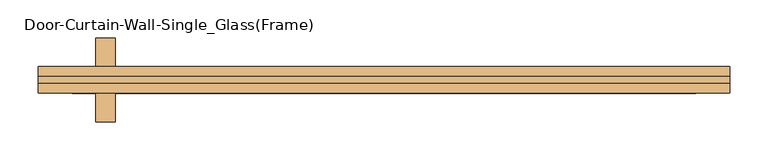
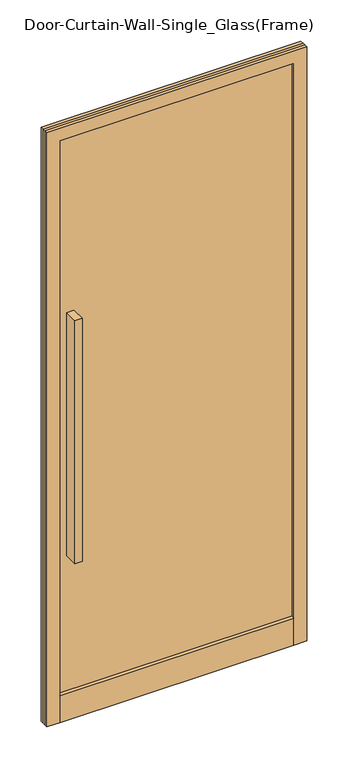
"""IFC4 building model written with IfcOpenShell, lengths in millimetres: door geometry, Door-Curtain-Wall-Single_Glass(Frame) : H_DR_AR B12_Door_Single_Glass_W1000xH2200_SSD-1."""

from ifc_helpers import new_model, si_unit, frame, origin, origin_with_axes, place, context, project, spatial, polyline, outline, extrude, source, transform, mapped, element, save


def door_curtain_wall_single_glass_frame_1226d56c(model_context):
    return source(origin(), model_context, "Body", "SweptSolid", [
        extrude(outline(polyline([(455.0, 0.0), (-455.0, 0.0), (-455.0, 9.0), (455.0, 9.0), (455.0, 0.0)])), origin_with_axes(), (0.0, 0.0, 1.0), 2200.0),
        extrude(outline(polyline([(-353.4, -50.8), (-378.8, -50.8), (-378.8, 0.0), (-353.4, 0.0), (-353.4, -50.8)])), frame((0.0, 0.0, 600.0), z_axis=(0.0, 0.0, 1.0), x_axis=(1.0, 0.0, 0.0)), (0.0, 0.0, 1.0), 900.0),
        extrude(outline(polyline([(-378.8, 59.8), (-353.4, 59.8), (-353.4, 9.0), (-378.8, 9.0), (-378.8, 59.8)])), frame((0.0, 0.0, 600.0), z_axis=(0.0, 0.0, 1.0), x_axis=(1.0, 0.0, 0.0)), (0.0, 0.0, 1.0), 900.0),
        extrude(outline(polyline([(0.0, 410.0), (0.0, 455.0), (2200.0, 455.0), (2200.0, -455.0), (0.0, -455.0), (0.0, -410.0), (2155.0, -410.0), (2155.0, 410.0), (0.0, 410.0)])), frame((0.0, -13.0, 0.0), z_axis=(0.0, 1.0, 0.0), x_axis=(0.0, 0.0, 1.0)), (0.0, 0.0, 1.0), 35.0),
        extrude(outline(polyline([(410.0, 22.0), (410.0, -13.0), (-410.0, -13.0), (-410.0, 22.0), (410.0, 22.0)])), origin_with_axes(), (0.0, 0.0, 1.0), 100.0),
    ])


if __name__ == "__main__":
    model = new_model("IFC4")
    model_context = context("Model", 3, world=origin())
    ifc_project = project(units=[si_unit("LENGTHUNIT", "METRE", prefix="MILLI")], contexts=[model_context])
    site = spatial("IfcSite", under=ifc_project)
    building = spatial("IfcBuilding", under=site)
    placement = place(None, origin())
    door_curtain_wall_single_glass_frame_shape = door_curtain_wall_single_glass_frame_1226d56c(model_context)
    element("IfcDoor", 1, ObjectType="Door-Curtain-Wall-Single_Glass(Frame) : H_DR_AR B12_Door_Single_Glass_W1000xH2200_SSD-1", at=placement, inside=building, context=model_context, shape_type="MappedRepresentation", body=[
        mapped(door_curtain_wall_single_glass_frame_shape, transform((0.0, 0.0, 0.0), x_axis=(1.0, 0.0, 0.0), y_axis=(0.0, 1.0, 0.0), z_axis=(0.0, 0.0, 1.0))),
    ])
    save(model, "model.ifc")

# Revit data of these elements
# Type "Door-Curtain-Wall-Single_Glass(Frame) : H_DR_AR B12_Door_Single_Glass_W1000xH2200_SSD-1"
#   Type Mark = "448"
#   Assembly Code = "B2030100"
#   Analytic Construction = "<None>"
#   Width [instance default] = 914.4 mm
#   Thermal Resistance (R) = 1.7611 (m²·K)/W
#   Swing Angle [instance default] = 90.00°
#   Frame Thk. = 45 mm
#   Frame_Thk2 = 100 mm
#   Heat Transfer Coefficient (U) = 0.567826 W/(m²·K)
#   Offset = 0 mm
#   Define Thermal Properties by = 1
#   Door Handle Material = 00_Metal_Stainless Steel
#   Glazing = 00_F_Glass
#   Visual Light Transmittance = 0
#   Solar Heat Gain Coefficient = 0
#   Construction Type Id = ""
#   Function = (empty or 0)
# Element 1 (IfcDoor, "Door-Curtain-Wall-Single_Glass(Frame) : H_DR_AR B12_Door_Single_Glass_W1000xH2200_SSD-1")
#   Width = 910 mm
#   Materials on its faces: "00_Metal_Stainless Steel", "00_F_Glass"
# Materials
#   "00_Metal_Stainless Steel": class "Metal", colour RGB 148 148 148, transparency 0, Description = "Steel", Cost = 0
#   "00_F_Glass": class "Glass", colour RGB 218 227 224, transparency 0.85, Description = "Glass", Cost = 0
